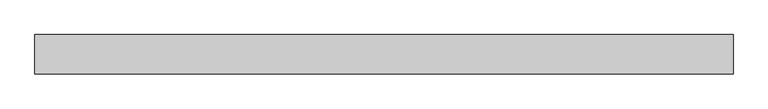
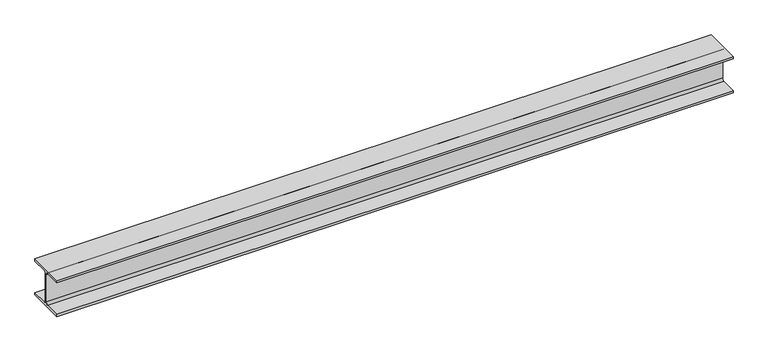
"""IFC4 building model written with IfcOpenShell, lengths in millimetres: beam geometry, 0912_Steel Framing_H-KSD3502 : H_SB_ASB_H-200x200x8x12."""

from ifc_helpers import new_model, si_unit, point, frame, frame_2d, origin, place, context, project, spatial, polyline, circle_curve, trimmed, segment, composite_curve, outline, extrude, source, transform, mapped, element, save


def beam_60b079e1(model_context):
    return source(origin(), model_context, "Body", "SweptSolid", [
        extrude(outline(composite_curve([segment(polyline([(100.0, -88.0), (100.0, -100.0), (-100.0, -100.0), (-100.0, -88.0), (-17.0, -88.0)]), True, "CONTINUOUS"), segment(trimmed(circle_curve(frame_2d((-17.0, -75.0)), 13.0), [point((-17.0, -88.0))], [point((-4.0, -75.0))], True, "CARTESIAN"), True, "CONTINUOUS"), segment(polyline([(-4.0, -75.0), (-4.0, 75.0)]), True, "CONTINUOUS"), segment(trimmed(circle_curve(frame_2d((-17.0, 75.0)), 13.0), [point((-4.0, 75.0))], [point((-17.0, 88.0))], True, "CARTESIAN"), True, "CONTINUOUS"), segment(polyline([(-17.0, 88.0), (-100.0, 88.0), (-100.0, 100.0), (100.0, 100.0), (100.0, 88.0), (17.0, 88.0)]), True, "CONTINUOUS"), segment(trimmed(circle_curve(frame_2d((17.0, 75.0)), 13.0), [point((17.0, 88.0))], [point((4.0, 75.0))], True, "CARTESIAN"), True, "CONTINUOUS"), segment(polyline([(4.0, 75.0), (4.0, -75.0)]), True, "CONTINUOUS"), segment(trimmed(circle_curve(frame_2d((17.0, -75.0)), 13.0), [point((4.0, -75.0))], [point((17.0, -88.0))], True, "CARTESIAN"), True, "CONTINUOUS"), segment(polyline([(17.0, -88.0), (100.0, -88.0)]), True, "CONTINUOUS")], self_intersect=False)), frame((-1842.2153264, 0.0, 0.0), z_axis=(1.0, 0.0, 0.0), x_axis=(0.0, 1.0, 0.0)), (0.0, 0.0, 1.0), 3556.4808254),
    ])


if __name__ == "__main__":
    model = new_model("IFC4")
    model_context = context("Model", 3, world=origin())
    ifc_project = project(units=[si_unit("LENGTHUNIT", "METRE", prefix="MILLI")], contexts=[model_context])
    site = spatial("IfcSite", under=ifc_project)
    building = spatial("IfcBuilding", under=site)
    placement = place(None, origin())
    beam_shape = beam_60b079e1(model_context)
    element("IfcBeam", 1, ObjectType="0912_Steel Framing_H-KSD3502 : H_SB_ASB_H-200x200x8x12", at=placement, inside=building, context=model_context, shape_type="MappedRepresentation", body=[
        mapped(beam_shape, transform((0.0, 0.0, 0.0), x_axis=(1.0, 0.0, 0.0), y_axis=(0.0, 1.0, 0.0), z_axis=(0.0, 0.0, 1.0))),
    ])
    save(model, "model.ifc")

# Revit data of these elements
# Type "0912_Steel Framing_H-KSD3502 : H_SB_ASB_H-200x200x8x12"
#   H_WM Code_1 = "S01AA002-00001 | Main Steel Structure Fabrication Work | Shelter/Building | Medium Steel - Standard (90KG/M>Weight≥30KG/M) | Material: (   )"
#   H_WM Code_2 = "S03AA028-00001 | Main Steel Structure Erection Work | Shelter/Building | Medium Steel (90KG/M>Weight≥30KG/M) | Material: (   )"
#   H_WM Code_3 = "S01AA010-00001 | Main Steel Structure Fabrication Work | Shelter/Building | Steel Painting/Coating | for Non-Fireproofed Steel Surface, Surface Preparation, Primer, Second & Final Coat | Material: (   )"
#   H_Q'ty Cal Type Tag = "SB-Q2"
#   Width = 20.0 cm
#   Web Thickness = 0.8 cm
#   Web Fillet = 1.3 cm
#   Warping Constant = 141000.0 cm⁶
#   W = 0
#   Torsional Moment of Inertia = 26.2485 cm⁴
#   Section Area = 63.53 cm²
#   Plastic Modulus weak axis = 244.0 cm³
#   Plastic Modulus strong axis = 525.0 cm³
#   Perimeter = 1.16 m²/m
#   Nominal Weight = 49.90 kgf/m
#   Moment of Inertia weak axis = 1600.00 cm⁴
#   Moment of Inertia strong axis = 4720.00 cm⁴
#   Height = 20.0 cm
#   Flange Thickness = 1.2 cm
#   Elastic Modulus weak axis = 160.0 cm³
#   Elastic Modulus strong axis = 472.0 cm³
#   Centroid Vertical = 10.0 cm
#   Centroid Horizontal = 10.0 cm
#   Ix = 47200000
#   Length [instance default] = 1.5240 m
#   Zx = 525000
#   b = 0.2000 m
#   h = 0.2000 m
#   r = 0.0130 m
#   s = 0.0080 m
#   t = 0.0120 m
#   A = 0.006353 m²
#   Structural Material [instance default] = Steel, 45-345
#   Assembly Code = ""
# Element 1 (IfcBeam, "0912_Steel Framing_H-KSD3502 : H_SB_ASB_H-200x200x8x12")
#   Structural Material = none
# Materials
#   "Steel, 45-345": class "Metal", colour RGB 189 187 185, transparency 0, Description = "Steel 345 MPa", Cost = 0
